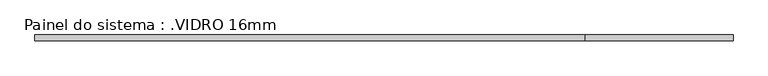
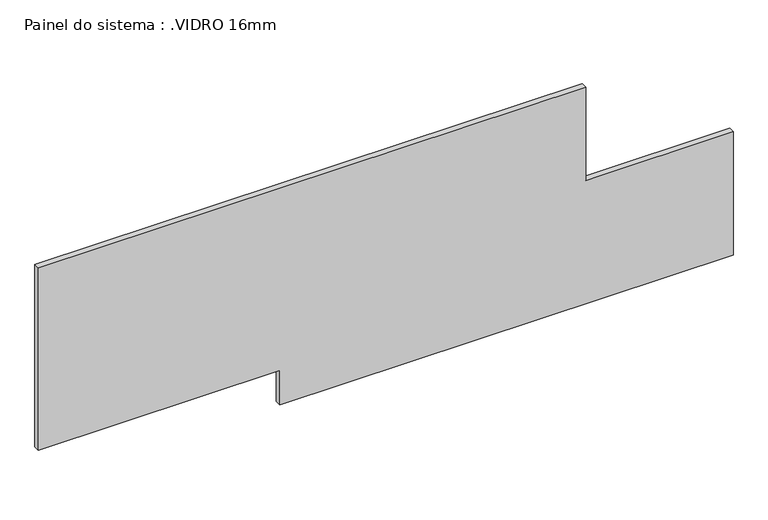
"""IFC4 building model written with IfcOpenShell, lengths in millimetres: plate geometry, Painel do sistema : .VIDRO 16mm."""

from ifc_helpers import new_model, si_unit, frame, origin, place, context, project, spatial, polyline, outline, extrude, source, transform, mapped, element, save


def painel_do_sistema_vidro_16mm_5f52dce1(model_context):
    return source(origin(), model_context, "Body", "SweptSolid", [
        extrude(outline(polyline([(0.0, -287.5), (0.0, 942.5), (353.3333333, 942.5), (353.3333333, 542.5), (621.6666667, 542.5), (621.6666667, -942.5), (98.3333333, -942.5), (98.3333333, -287.5), (0.0, -287.5)])), frame((0.0, -200.0, 0.0), z_axis=(0.0, 1.0, 0.0), x_axis=(0.0, 0.0, 1.0)), (0.0, 0.0, 1.0), 16.0),
    ])


if __name__ == "__main__":
    model = new_model("IFC4")
    model_context = context("Model", 3, world=origin())
    ifc_project = project(units=[si_unit("LENGTHUNIT", "METRE", prefix="MILLI")], contexts=[model_context])
    site = spatial("IfcSite", under=ifc_project)
    building = spatial("IfcBuilding", under=site)
    placement = place(None, origin())
    painel_do_sistema_vidro_16mm_shape = painel_do_sistema_vidro_16mm_5f52dce1(model_context)
    element("IfcPlate", 1, ObjectType="Painel do sistema : .VIDRO 16mm", at=placement, inside=building, context=model_context, shape_type="MappedRepresentation", body=[
        mapped(painel_do_sistema_vidro_16mm_shape, transform((0.0, 0.0, 0.0), x_axis=(1.0, 0.0, 0.0), y_axis=(0.0, 1.0, 0.0), z_axis=(0.0, 0.0, 1.0))),
    ])
    save(model, "model.ifc")

# Revit data of these elements
# Element 1 (IfcPlate, "Painel do sistema : .VIDRO 16mm")
#   Materials on its faces: ".VIDRO"
# Materials
#   ".VIDRO": class "Genérico", colour RGB 198 236 255, transparency 0.95, Cost = 0
